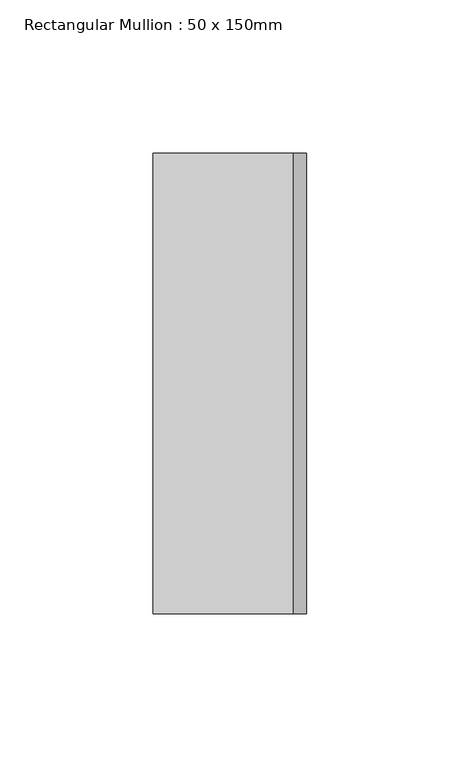
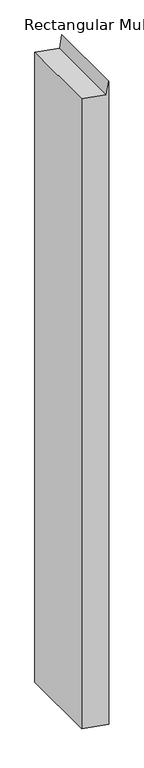
"""IFC4 building model written with IfcOpenShell, lengths in millimetres: member geometry, Rectangular Mullion : 50 x 150mm."""

from ifc_helpers import new_model, si_unit, frame, origin, place, context, project, spatial, polyline, outline, extrude, source, transform, mapped, element, save


def rectangular_mullion_50_x_150mm_4ea697b8(model_context):
    return source(origin(), model_context, "Body", "SweptSolid", [
        extrude(outline(polyline([(25.0, 0.0), (0.3798062, -4.3412044), (8.4306837, -50.0), (-1222.9211547, -50.0), (-1231.7375037, 0.0), (25.0, 0.0)])), frame((0.0, -75.0, 0.0), z_axis=(0.0, 1.0, 0.0), x_axis=(0.0, 0.0, 1.0)), (0.0, 0.0, 1.0), 150.0),
    ])


if __name__ == "__main__":
    model = new_model("IFC4")
    model_context = context("Model", 3, world=origin())
    ifc_project = project(units=[si_unit("LENGTHUNIT", "METRE", prefix="MILLI")], contexts=[model_context])
    site = spatial("IfcSite", under=ifc_project)
    building = spatial("IfcBuilding", under=site)
    placement = place(None, origin())
    rectangular_mullion_50_x_150mm_shape = rectangular_mullion_50_x_150mm_4ea697b8(model_context)
    element("IfcMember", 1, ObjectType="Rectangular Mullion : 50 x 150mm", at=placement, inside=building, context=model_context, shape_type="MappedRepresentation", body=[
        mapped(rectangular_mullion_50_x_150mm_shape, transform((0.0, 0.0, 0.0), x_axis=(1.0, 0.0, 0.0), y_axis=(0.0, 1.0, 0.0), z_axis=(0.0, 0.0, 1.0))),
    ])
    save(model, "model.ifc")

# Revit data of these elements
# Type "Rectangular Mullion : 50 x 150mm"
#   built-in parameter 1007304 = 0.492126 (stored number, unit not read)
#   built-in parameter 1007301 = 0.082021 (stored number, unit not read)
#   built-in parameter 1007300 = 0.082021 (stored number, unit not read)
# Element 1 (IfcMember, "Rectangular Mullion : 50 x 150mm")
#   Materials on its faces: "Aluminium"
# Materials
#   "Aluminium": class "Metal", colour RGB 247 247 247, transparency 0, Description = "Aluminium 6061", Cost = 0
